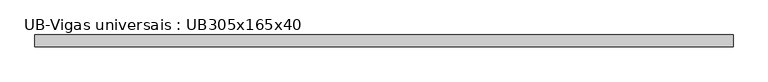
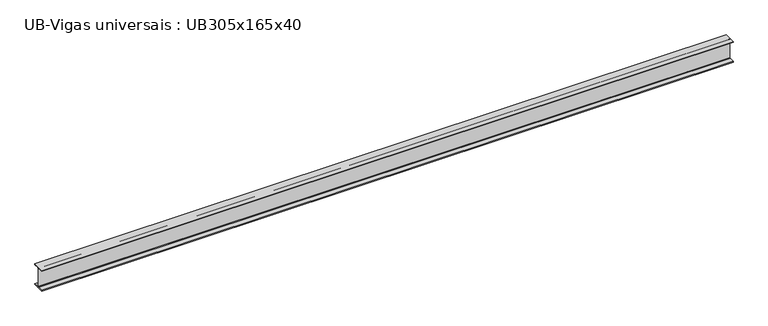
"""IFC4 building model written with IfcOpenShell, lengths in millimetres: beam geometry, UB-Vigas universais : UB305x165x40."""

from ifc_helpers import new_model, si_unit, point, frame, frame_2d, origin, place, context, project, spatial, polyline, circle_curve, trimmed, segment, composite_curve, outline, extrude, source, transform, mapped, element, save


def ub_vigas_universais_ub305x165x40_b8b89153(model_context):
    return source(origin(), model_context, "Body", "SweptSolid", [
        extrude(outline(composite_curve([segment(polyline([(82.5, -141.5), (82.5, -151.7), (-82.5, -151.7), (-82.5, -141.5), (-11.9, -141.5)]), True, "CONTINUOUS"), segment(trimmed(circle_curve(frame_2d((-11.9, -132.6)), 8.9), [point((-11.9, -141.5))], [point((-3.0, -132.6))], True, "CARTESIAN"), True, "CONTINUOUS"), segment(polyline([(-3.0, -132.6), (-3.0, 132.6)]), True, "CONTINUOUS"), segment(trimmed(circle_curve(frame_2d((-11.9, 132.6)), 8.9), [point((-3.0, 132.6))], [point((-11.9, 141.5))], True, "CARTESIAN"), True, "CONTINUOUS"), segment(polyline([(-11.9, 141.5), (-82.5, 141.5), (-82.5, 151.7), (82.5, 151.7), (82.5, 141.5), (11.9, 141.5)]), True, "CONTINUOUS"), segment(trimmed(circle_curve(frame_2d((11.9, 132.6)), 8.9), [point((11.9, 141.5))], [point((3.0, 132.6))], True, "CARTESIAN"), True, "CONTINUOUS"), segment(polyline([(3.0, 132.6), (3.0, -132.6)]), True, "CONTINUOUS"), segment(trimmed(circle_curve(frame_2d((11.9, -132.6)), 8.9), [point((3.0, -132.6))], [point((11.9, -141.5))], True, "CARTESIAN"), True, "CONTINUOUS"), segment(polyline([(11.9, -141.5), (82.5, -141.5)]), True, "CONTINUOUS")], self_intersect=False)), frame((-4862.3, 0.0, 0.0), z_axis=(1.0, 0.0, 0.0), x_axis=(0.0, 1.0, 0.0)), (0.0, 0.0, 1.0), 9724.6),
    ])


if __name__ == "__main__":
    model = new_model("IFC4")
    model_context = context("Model", 3, world=origin())
    ifc_project = project(units=[si_unit("LENGTHUNIT", "METRE", prefix="MILLI")], contexts=[model_context])
    site = spatial("IfcSite", under=ifc_project)
    building = spatial("IfcBuilding", under=site)
    placement = place(None, origin())
    ub_vigas_universais_ub305x165x40_shape = ub_vigas_universais_ub305x165x40_b8b89153(model_context)
    element("IfcBeam", 1, ObjectType="UB-Vigas universais : UB305x165x40", at=placement, inside=building, context=model_context, shape_type="MappedRepresentation", body=[
        mapped(ub_vigas_universais_ub305x165x40_shape, transform((0.0, 0.0, 0.0), x_axis=(1.0, 0.0, 0.0), y_axis=(0.0, 1.0, 0.0), z_axis=(0.0, 0.0, 1.0))),
    ])
    save(model, "model.ifc")

# Revit data of these elements
# Type "UB-Vigas universais : UB305x165x40"
#   Section Name Key = "UB305X165X40"
#   Width = 16.5 cm
#   Web Thickness = 0.6 cm
#   Web Fillet = 0.89 cm
#   Warping Constant = 164000.0 cm⁶
#   Torsional Moment of Inertia = 14.70 cm⁴
#   Section Area = 51.3 cm²
#   Plastic Modulus weak axis = 142.0 cm³
#   Plastic Modulus strong axis = 623.0 cm³
#   Nominal Weight = 40.2999 kgf/m
#   Moment of Inertia weak axis = 764.00 cm⁴
#   Moment of Inertia strong axis = 8503.00 cm⁴
#   Height = 30.34 cm
#   Flange Thickness = 1.02 cm
#   Elastic Modulus weak axis = 92.6 cm³
#   Elastic Modulus strong axis = 560.0 cm³
#   Centroid Vertical = 15.17 cm
#   Centroid Horizontal = 8.25 cm
#   Length [instance default] = 1.50 m
#   Structural Material [instance default] = Metal - Aço 43-275
#   Type Comments = ""
#   Assembly Code = ""
# Element 1 (IfcBeam, "UB-Vigas universais : UB305x165x40")
#   Materials on its faces: "Metal - Aço 43-275"
# Materials
#   "Metal - Aço 43-275": class "Metal", colour RGB 247 247 247, transparency 0, Cost = 0
